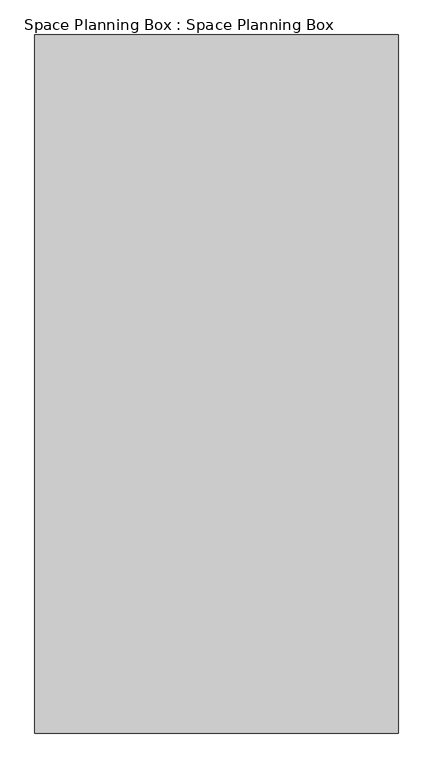
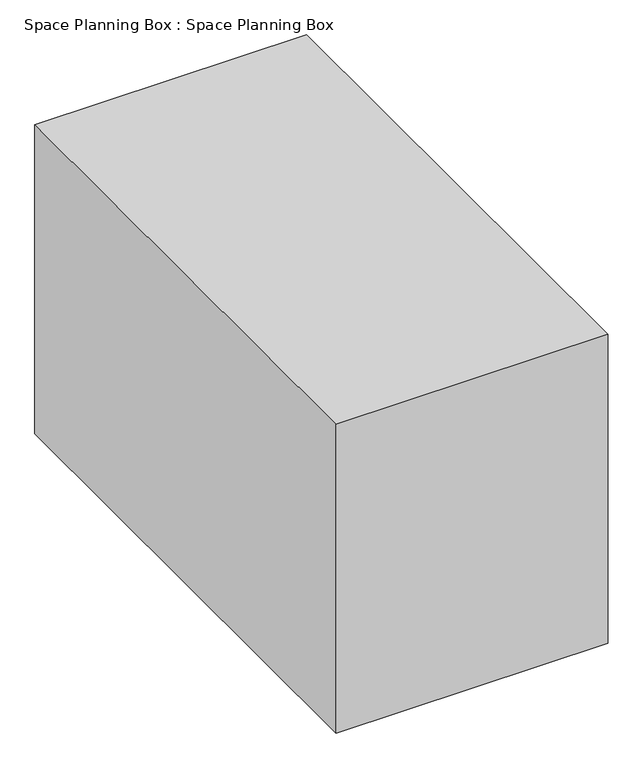
"""IFC4 building model written with IfcOpenShell, lengths in millimetres: proxy geometry, Space Planning Box : Space Planning Box."""

from ifc_helpers import new_model, si_unit, origin, origin_with_axes, place, context, project, spatial, polyline, outline, extrude, source, transform, mapped, element, save


def space_planning_box_space_planning_box_7902148a(model_context):
    return source(origin(), model_context, "Body", "SweptSolid", [
        extrude(outline(polyline([(2500.0, 4800.0), (2500.0, -4800.0), (-2500.0, -4800.0), (-2500.0, 4800.0), (2500.0, 4800.0)])), origin_with_axes(), (0.0, 0.0, 1.0), 6000.0),
    ])


if __name__ == "__main__":
    model = new_model("IFC4")
    model_context = context("Model", 3, world=origin())
    ifc_project = project(units=[si_unit("LENGTHUNIT", "METRE", prefix="MILLI")], contexts=[model_context])
    site = spatial("IfcSite", under=ifc_project)
    building = spatial("IfcBuilding", under=site)
    placement = place(None, origin())
    space_planning_box_space_planning_box_shape = space_planning_box_space_planning_box_7902148a(model_context)
    element("IfcBuildingElementProxy", 1, Name="Space Planning Box : Space Planning Box", ObjectType="Space Planning Box : Space Planning Box", at=placement, inside=building, context=model_context, shape_type="MappedRepresentation", body=[
        mapped(space_planning_box_space_planning_box_shape, transform((0.0, 0.0, 0.0), x_axis=(1.0, 0.0, 0.0), y_axis=(0.0, 1.0, 0.0), z_axis=(0.0, 0.0, 1.0))),
    ])
    save(model, "model.ifc")

# Revit data of these elements
# Type "Space Planning Box : Space Planning Box"
#   Type Comments = "..."
#   Room Name [instance default] = "?"
#   Assembly Code = "..."
#   Width [instance default] = 1524 mm
#   Program Area [instance default] = 0 m²
#   Length [instance default] = 1524 mm
#   Height [instance default] = 1524 mm
#   Area [instance default] = 2.32258 m²
#   Fill Color [instance default] = Cyan
#   Default Elevation = 0
# Element 1 (IfcBuildingElementProxy, "Space Planning Box : Space Planning Box")
#   Room Name = "Document Room"
#   Width = 5000 mm
#   Program Area = 48 m²
#   Length = 9600 mm
#   Height = 6000 mm
#   Area = 48 m²
#   Fill Color = Lavender
#   Materials on its faces: "Lavender"
# Materials
#   "Cyan": class "Generic", colour RGB 0 255 255, transparency 0.2, Cost = 0
#   "Lavender": class "Generic", colour RGB 186 85 211, transparency 0.2, Cost = 0
